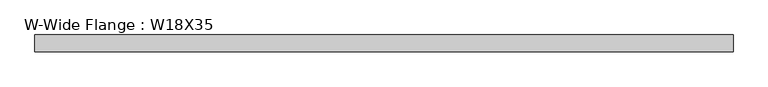
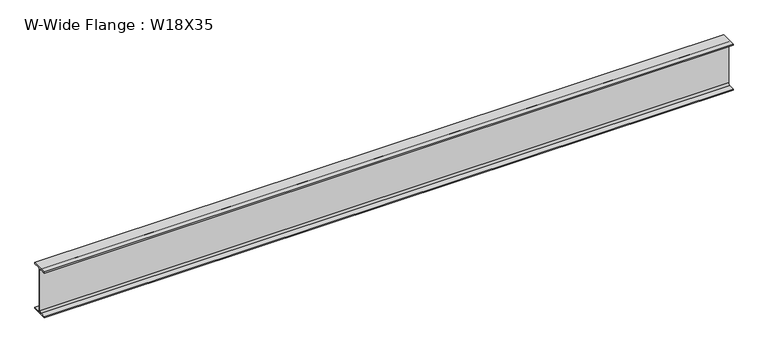
"""IFC4 building model written with IfcOpenShell, lengths in millimetres: beam geometry, W-Wide Flange : W18X35."""

from ifc_helpers import new_model, si_unit, point, frame, frame_2d, origin, place, context, project, spatial, polyline, circle_curve, trimmed, segment, composite_curve, outline, extrude, source, transform, mapped, element, save


def w_wide_flange_w18x35_9e390736(model_context):
    return source(origin(), model_context, "Body", "SweptSolid", [
        extrude(outline(composite_curve([segment(polyline([(-76.2, -213.995), (-21.59, -213.995)]), True, "CONTINUOUS"), segment(trimmed(circle_curve(frame_2d((-21.59, -196.215)), 17.78), [point((-21.59, -213.995))], [point((-3.81, -196.215))], True, "CARTESIAN"), True, "CONTINUOUS"), segment(polyline([(-3.81, -196.215), (-3.81, 196.215)]), True, "CONTINUOUS"), segment(trimmed(circle_curve(frame_2d((-21.59, 196.215)), 17.78), [point((-3.81, 196.215))], [point((-21.59, 213.995))], True, "CARTESIAN"), True, "CONTINUOUS"), segment(polyline([(-21.59, 213.995), (-76.2, 213.995), (-76.2, 224.79), (76.2, 224.79), (76.2, 213.995), (21.59, 213.995)]), True, "CONTINUOUS"), segment(trimmed(circle_curve(frame_2d((21.59, 196.215)), 17.78), [point((21.59, 213.995))], [point((3.81, 196.215))], True, "CARTESIAN"), True, "CONTINUOUS"), segment(polyline([(3.81, 196.215), (3.81, -196.215)]), True, "CONTINUOUS"), segment(trimmed(circle_curve(frame_2d((21.59, -196.215)), 17.78), [point((3.81, -196.215))], [point((21.59, -213.995))], True, "CARTESIAN"), True, "CONTINUOUS"), segment(polyline([(21.59, -213.995), (76.2, -213.995), (76.2, -224.79), (-76.2, -224.79), (-76.2, -213.995)]), True, "CONTINUOUS")], self_intersect=False)), frame((-3162.8437614, 0.0, 0.0), z_axis=(1.0, 0.0, 0.0), x_axis=(0.0, 1.0, 0.0)), (0.0, 0.0, 1.0), 6366.51),
    ])


if __name__ == "__main__":
    model = new_model("IFC4")
    model_context = context("Model", 3, world=origin())
    ifc_project = project(units=[si_unit("LENGTHUNIT", "METRE", prefix="MILLI")], contexts=[model_context])
    site = spatial("IfcSite", under=ifc_project)
    building = spatial("IfcBuilding", under=site)
    placement = place(None, origin())
    w_wide_flange_w18x35_shape = w_wide_flange_w18x35_9e390736(model_context)
    element("IfcBeam", 1, ObjectType="W-Wide Flange : W18X35", at=placement, inside=building, context=model_context, shape_type="MappedRepresentation", body=[
        mapped(w_wide_flange_w18x35_shape, transform((0.0, 0.0, 0.0), x_axis=(1.0, 0.0, 0.0), y_axis=(0.0, 1.0, 0.0), z_axis=(0.0, 0.0, 1.0))),
    ])
    save(model, "model.ifc")

# Revit data of these elements
# Type "W-Wide Flange : W18X35"
#   Assembly Code = "B10"
#   W = 35
#   Start Extension Calculation [instance default] = 10' - 0"
#   Start Extension [instance default] = -0' - 0 1/2"
#   End Extension Calculation [instance default] = 10' - 0"
#   End Extension [instance default] = -0' - 0 1/2"
#   Length [instance default] = 5' - 0"
#   bf = 0' - 6"
#   d = 1' - 5.7"
#   k = 0' - 1 1/8"
#   k2 = 0' - 0.7"
#   tf = 0' - 0.425"
#   tw = 0' - 0.3"
#   A = 0.0715278 SF
#   Beam Material [instance default] = Metal - Steel - ASTM A992
# Element 1 (IfcBeam, "W-Wide Flange : W18X35")
#   Materials on its faces: "Metal - Steel - ASTM A992"
# Materials
#   "Metal - Steel - ASTM A992": class "Metal", colour RGB 128 0 0, transparency 0
